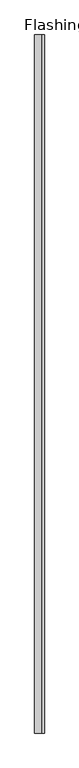
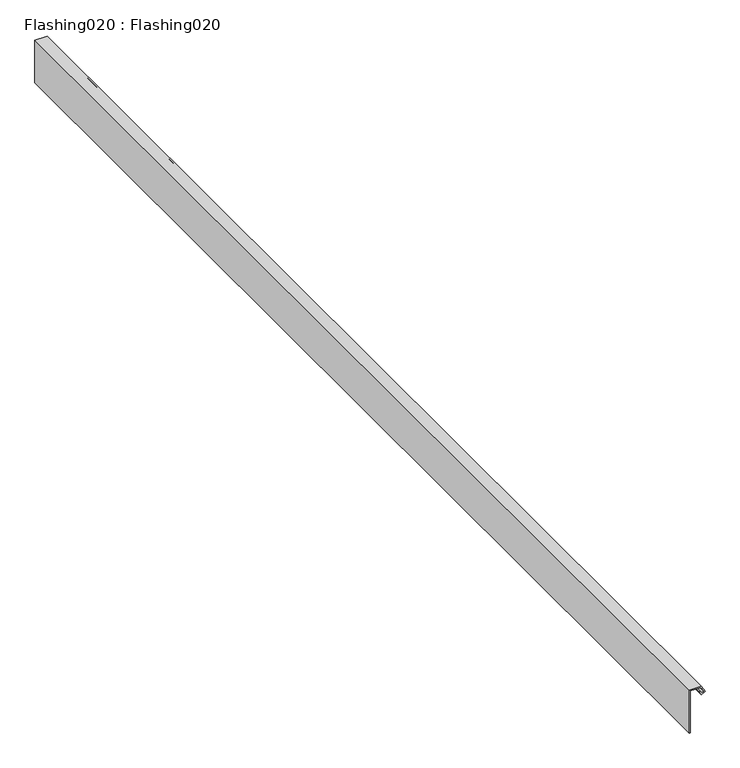
"""IFC4 building model written with IfcOpenShell, lengths in millimetres: proxy geometry, Flashing020 : Flashing020."""

from ifc_helpers import new_model, si_unit, frame, origin, place, context, project, spatial, polyline, outline, extrude, source, transform, mapped, element, save


def flashing020_flashing020_07dce5c2(model_context):
    return source(origin(), model_context, "Body", "SweptSolid", [
        extrude(outline(polyline([(40707.8367188, 16632.328125), (40785.71875, 16632.328125), (40785.71875, 16650.5221509), (40777.2623654, 16655.298745), (40775.2340727, 16652.1607025), (40779.327926, 16649.9538597), (40778.3789063, 16648.1933594), (40772.3789063, 16651.4277344), (40776.6054688, 16657.9667969), (40787.71875, 16651.6894531), (40787.71875, 16630.328125), (40707.8367188, 16630.328125), (40707.8367188, 16632.328125)])), frame((0.0, 7982.1449112, 0.0), z_axis=(0.0, 1.0, 0.0), x_axis=(0.0, 0.0, 1.0)), (0.0, 0.0, 1.0), 2000.0),
    ])


if __name__ == "__main__":
    model = new_model("IFC4")
    model_context = context("Model", 3, world=origin())
    ifc_project = project(units=[si_unit("LENGTHUNIT", "METRE", prefix="MILLI")], contexts=[model_context])
    site = spatial("IfcSite", under=ifc_project)
    building = spatial("IfcBuilding", under=site)
    placement = place(None, origin())
    flashing020_flashing020_shape = flashing020_flashing020_07dce5c2(model_context)
    element("IfcBuildingElementProxy", 1, Name="Flashing020 : Flashing020", ObjectType="Flashing020 : Flashing020", at=placement, inside=building, context=model_context, shape_type="MappedRepresentation", body=[
        mapped(flashing020_flashing020_shape, transform((0.0, 0.0, 0.0), x_axis=(1.0, 0.0, 0.0), y_axis=(0.0, 1.0, 0.0), z_axis=(0.0, 0.0, 1.0))),
    ])
    save(model, "model.ifc")

# Revit data of these elements
# Type "Flashing020 : Flashing020"
#   NameOverride = "Flashing020"
# Element 1 (IfcBuildingElementProxy, "Flashing020 : Flashing020")
#   Materials on its faces: "BRAKE METAL TO WRAP FRAMING OVER BITUTHANE"
# Materials
#   "BRAKE METAL TO WRAP FRAMING OVER BITUTHANE": class "Unassigned", colour RGB 128 128 128, transparency 0, Cost = 0
